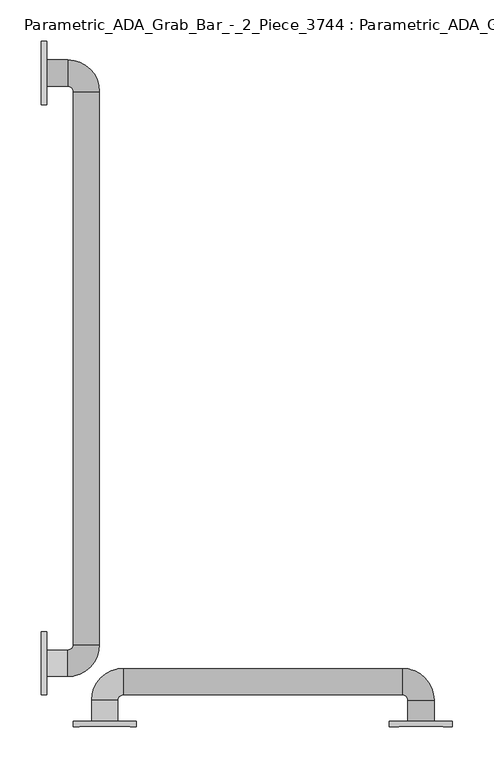
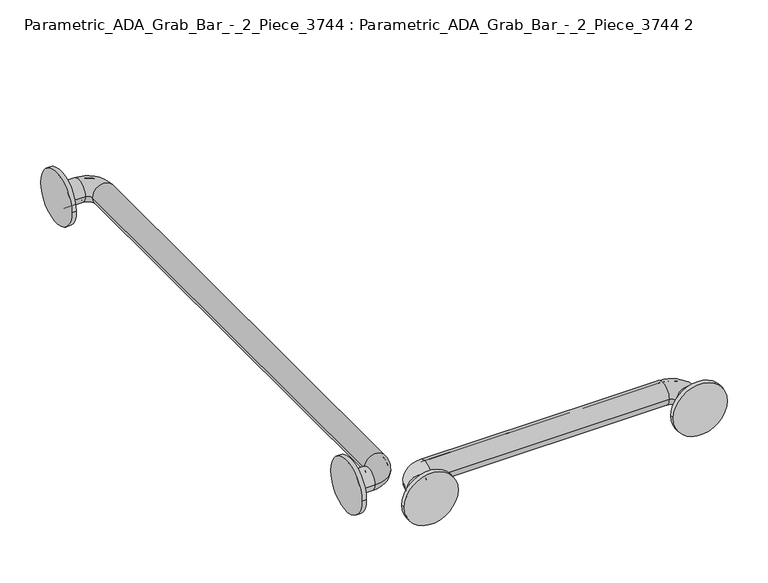
"""IFC4 building model written with IfcOpenShell, lengths in millimetres: proxy geometry, Parametric_ADA_Grab_Bar_-_2_Piece_3744 : Parametric_ADA_Grab_Bar_-_2_Piece_3744 2."""

from ifc_helpers import new_model, si_unit, point, frame, frame_2d, origin, place, context, project, spatial, polyline, circle_curve, ellipse_curve, trimmed, segment, composite_curve, outline, extrude, source, transform, mapped, element, save
from ifc_brep_helpers import plane_surface, cylinder_surface, revolved_surface, advanced_brep


def parametric_ada_grab_bar_2_piece_3744_parametric_ada_grab_bar_cda52879(model_context):
    return source(origin(), model_context, "Body", "SolidModel", [
        advanced_brep(
        [(6.35, 785.01875, 838.2), (6.35, 816.76875, 838.2), (6.35, 788.19375, 838.2), (6.35, 813.59375, 838.2), (31.75, 785.01875, 838.2), (31.75, 816.76875, 838.2), (31.75, 788.19375, 838.2), (31.75, 813.59375, 838.2), (69.85, 778.66875, 838.2), (38.1, 778.66875, 838.2), (66.675, 778.66875, 838.2), (41.275, 778.66875, 838.2), (38.1, 111.91875, 838.2), (69.85, 111.91875, 838.2), (41.275, 111.91875, 838.2), (66.675, 111.91875, 838.2), (31.75, 73.81875, 838.2), (31.75, 105.56875, 838.2), (31.75, 76.99375, 838.2), (31.75, 102.39375, 838.2), (6.35, 105.56875, 838.2), (6.35, 73.81875, 838.2), (6.35, 102.39375, 838.2), (6.35, 76.99375, 838.2)],
        [
            (0, 1, circle_curve(frame((6.35, 800.89375, 838.2), z_axis=(-1.0, 0.0, 0.0), x_axis=(0.0, 1.0, 0.0)), 15.875)),
            (1, 0, circle_curve(frame((6.35, 800.89375, 838.2), z_axis=(-1.0, 0.0, 0.0), x_axis=(0.0, 1.0, 0.0)), 15.875)),
            (2, 3, circle_curve(frame((6.35, 800.89375, 838.2), z_axis=(1.0, 0.0, 0.0), x_axis=(0.0, 1.0, 0.0)), 12.7)),
            (3, 2, circle_curve(frame((6.35, 800.89375, 838.2), z_axis=(1.0, 0.0, 0.0), x_axis=(0.0, 1.0, 0.0)), 12.7)),
            (0, 4),
            (4, 5, circle_curve(frame((31.75, 800.89375, 838.2), z_axis=(-1.0, 0.0, 0.0), x_axis=(0.0, 1.0, 0.0)), 15.875)),
            (5, 1),
            (5, 4, circle_curve(frame((31.75, 800.89375, 838.2), z_axis=(-1.0, 0.0, 0.0), x_axis=(0.0, 1.0, 0.0)), 15.875)),
            (2, 6),
            (6, 7, circle_curve(frame((31.75, 800.89375, 838.2), z_axis=(1.0, 0.0, 0.0), x_axis=(0.0, 1.0, 0.0)), 12.7)),
            (7, 3),
            (7, 6, circle_curve(frame((31.75, 800.89375, 838.2), z_axis=(1.0, 0.0, 0.0), x_axis=(0.0, 1.0, 0.0)), 12.7)),
            (8, 5, circle_curve(frame((31.75, 778.66875, 838.2), z_axis=(0.0, 0.0, 1.0), x_axis=(0.0, 1.0, 0.0)), 38.1)),
            (4, 9, circle_curve(frame((31.75, 778.66875, 838.2), z_axis=(0.0, 0.0, -1.0), x_axis=(0.0, 1.0, 0.0)), 6.35)),
            (9, 8, circle_curve(frame((53.975, 778.66875, 838.2), z_axis=(0.0, 1.0, 0.0), x_axis=(1.0, 0.0, 0.0)), 15.875)),
            (8, 9, circle_curve(frame((53.975, 778.66875, 838.2), z_axis=(0.0, 1.0, 0.0), x_axis=(1.0, 0.0, 0.0)), 15.875)),
            (10, 7, circle_curve(frame((31.75, 778.66875, 838.2), z_axis=(0.0, 0.0, 1.0), x_axis=(0.0, 1.0, 0.0)), 34.925)),
            (6, 11, circle_curve(frame((31.75, 778.66875, 838.2), z_axis=(0.0, 0.0, -1.0), x_axis=(0.0, 1.0, 0.0)), 9.525)),
            (11, 10, circle_curve(frame((53.975, 778.66875, 838.2), z_axis=(0.0, -1.0, 0.0), x_axis=(1.0, 0.0, 0.0)), 12.7)),
            (10, 11, circle_curve(frame((53.975, 778.66875, 838.2), z_axis=(0.0, -1.0, 0.0), x_axis=(1.0, 0.0, 0.0)), 12.7)),
            (9, 12),
            (12, 13, circle_curve(frame((53.975, 111.91875, 838.2), z_axis=(0.0, 1.0, 0.0), x_axis=(1.0, 0.0, 0.0)), 15.875)),
            (13, 8),
            (13, 12, circle_curve(frame((53.975, 111.91875, 838.2), z_axis=(0.0, 1.0, 0.0), x_axis=(1.0, 0.0, 0.0)), 15.875)),
            (11, 14),
            (14, 15, circle_curve(frame((53.975, 111.91875, 838.2), z_axis=(0.0, -1.0, 0.0), x_axis=(1.0, 0.0, 0.0)), 12.7)),
            (15, 10),
            (15, 14, circle_curve(frame((53.975, 111.91875, 838.2), z_axis=(0.0, -1.0, 0.0), x_axis=(1.0, 0.0, 0.0)), 12.7)),
            (16, 13, circle_curve(frame((31.75, 111.91875, 838.2), z_axis=(0.0, 0.0, 1.0), x_axis=(1.0, 0.0, 0.0)), 38.1)),
            (12, 17, circle_curve(frame((31.75, 111.91875, 838.2), z_axis=(0.0, 0.0, -1.0), x_axis=(1.0, 0.0, 0.0)), 6.35)),
            (17, 16, circle_curve(frame((31.75, 89.69375, 838.2), z_axis=(1.0, -1.076610172186615e-12, 0.0), x_axis=(-1.076610172186615e-12, -1.0, 0.0)), 15.875)),
            (16, 17, circle_curve(frame((31.75, 89.69375, 838.2), z_axis=(1.0, 0.0, 0.0), x_axis=(0.0, -1.0, 0.0)), 15.875)),
            (18, 15, circle_curve(frame((31.75, 111.91875, 838.2), z_axis=(0.0, 0.0, 1.0), x_axis=(1.0, 0.0, 0.0)), 34.925)),
            (14, 19, circle_curve(frame((31.75, 111.91875, 838.2), z_axis=(0.0, 0.0, -1.0), x_axis=(1.0, 0.0, 0.0)), 9.525)),
            (19, 18, circle_curve(frame((31.75, 89.69375, 838.2), z_axis=(-1.0, 0.0, 0.0), x_axis=(0.0, -1.0, 0.0)), 12.7)),
            (18, 19, circle_curve(frame((31.75, 89.69375, 838.2), z_axis=(-1.0, 0.0, 0.0), x_axis=(0.0, -1.0, 0.0)), 12.7)),
            (20, 21, circle_curve(frame((6.35, 89.69375, 838.2), z_axis=(-1.0, 0.0, 0.0), x_axis=(0.0, -1.0, 0.0)), 15.875)),
            (21, 20, circle_curve(frame((6.35, 89.69375, 838.2), z_axis=(-1.0, 0.0, 0.0), x_axis=(0.0, -1.0, 0.0)), 15.875)),
            (22, 23, circle_curve(frame((6.35, 89.69375, 838.2), z_axis=(1.0, 0.0, 0.0), x_axis=(0.0, -1.0, 0.0)), 12.7)),
            (23, 22, circle_curve(frame((6.35, 89.69375, 838.2), z_axis=(1.0, 0.0, 0.0), x_axis=(0.0, -1.0, 0.0)), 12.7)),
            (17, 20),
            (21, 16),
            (19, 22),
            (23, 18),
        ],
        [
            plane_surface(frame((6.35, 800.89375, 838.2), z_axis=(-1.0, 0.0, 0.0), x_axis=(0.0, 0.0, 1.0))),
            cylinder_surface(frame((6.35, 800.89375, 838.2), z_axis=(-1.0, 0.0, 0.0), x_axis=(0.0, 1.0, 0.0)), 15.875),
            revolved_surface(polyline([(31.75, 813.59375, 838.2), (6.35, 813.59375, 838.2)]), (6.35, 800.89375, 838.2), (1.0, 0.0, 0.0)),
            revolved_surface(trimmed(ellipse_curve(frame((31.75, 800.89375, 838.2), z_axis=(-1.0, 0.0, 0.0), x_axis=(0.0, 1.0, 0.0)), 15.875, 15.875), [point((31.75, 785.01875, 838.2))], [point((31.75, 816.76875, 838.2))], True, "CARTESIAN"), (31.75, 778.66875, 838.2), (0.0, 0.0, -1.0)),
            revolved_surface(trimmed(ellipse_curve(frame((31.75, 800.89375, 838.2), z_axis=(-1.0, 0.0, 0.0), x_axis=(0.0, 1.0, 0.0)), 15.875, 15.875), [point((31.75, 816.76875, 838.2))], [point((31.75, 785.01875, 838.2))], True, "CARTESIAN"), (31.75, 778.66875, 838.2), (0.0, 0.0, -1.0)),
            revolved_surface(trimmed(ellipse_curve(frame((31.75, 800.89375, 838.2), z_axis=(1.0, 0.0, 0.0), x_axis=(0.0, 1.0, 0.0)), 12.7, 12.7), [point((31.75, 788.19375, 838.2))], [point((31.75, 813.59375, 838.2))], True, "CARTESIAN"), (31.75, 778.66875, 838.2), (0.0, 0.0, -1.0)),
            revolved_surface(trimmed(ellipse_curve(frame((31.75, 800.89375, 838.2), z_axis=(1.0, 0.0, 0.0), x_axis=(0.0, 1.0, 0.0)), 12.7, 12.7), [point((31.75, 813.59375, 838.2))], [point((31.75, 788.19375, 838.2))], True, "CARTESIAN"), (31.75, 778.66875, 838.2), (0.0, 0.0, -1.0)),
            cylinder_surface(frame((53.975, 778.66875, 838.2), z_axis=(0.0, 1.0, 0.0), x_axis=(1.0, 0.0, 0.0)), 15.875),
            revolved_surface(polyline([(66.675, 111.91875000000005, 838.2), (66.675, 778.66875, 838.2)]), (53.975, 778.66875, 838.2), (0.0, -1.0, 0.0)),
            revolved_surface(trimmed(ellipse_curve(frame((53.975, 111.91875, 838.2), z_axis=(0.0, 1.0, 0.0), x_axis=(1.0, 0.0, 0.0)), 15.875, 15.875), [point((38.1, 111.91875, 838.2))], [point((69.85, 111.91875, 838.2))], True, "CARTESIAN"), (31.75, 111.91875, 838.2), (0.0, 0.0, -1.0)),
            revolved_surface(trimmed(ellipse_curve(frame((53.975, 111.91875, 838.2), z_axis=(0.0, 1.0, 0.0), x_axis=(1.0, 0.0, 0.0)), 15.875, 15.875), [point((69.85, 111.91875, 838.2))], [point((38.1, 111.91875, 838.2))], True, "CARTESIAN"), (31.75, 111.91875, 838.2), (0.0, 0.0, -1.0)),
            revolved_surface(trimmed(ellipse_curve(frame((53.975, 111.91875, 838.2), z_axis=(0.0, -1.0, 0.0), x_axis=(1.0, 0.0, 0.0)), 12.7, 12.7), [point((41.275, 111.91875, 838.2))], [point((66.675, 111.91875, 838.2))], True, "CARTESIAN"), (31.75, 111.91875, 838.2), (0.0, 0.0, -1.0)),
            revolved_surface(trimmed(ellipse_curve(frame((53.975, 111.91875, 838.2), z_axis=(0.0, -1.0, 0.0), x_axis=(1.0, 0.0, 0.0)), 12.7, 12.7), [point((66.675, 111.91875, 838.2))], [point((41.275, 111.91875, 838.2))], True, "CARTESIAN"), (31.75, 111.91875, 838.2), (0.0, 0.0, -1.0)),
            plane_surface(frame((6.35, 89.69375, 838.2), z_axis=(-1.0, 0.0, 0.0), x_axis=(0.0, 0.0, 1.0))),
            cylinder_surface(frame((31.75, 89.69375, 838.2), z_axis=(1.0, 0.0, 0.0), x_axis=(0.0, -1.0, 0.0)), 15.875),
            revolved_surface(polyline([(6.350000000000001, 76.99374999999999, 838.2), (31.75, 76.99374999999999, 838.2)]), (31.75, 89.69375, 838.2), (-1.0, 0.0, 0.0)),
        ],
        [
            (0, [[1, 2], [3, 4]]),
            (1, [[-1, 5, 6, 7]]),
            (1, [[-2, -7, 8, -5]]),
            (2, [[-3, 9, 10, 11]]),
            (2, [[-4, -11, 12, -9]]),
            (3, [[13, -6, 14, 15]]),
            (4, [[-14, -8, -13, 16]]),
            (5, [[17, -10, 18, 19]]),
            (6, [[-18, -12, -17, 20]]),
            (7, [[-15, 21, 22, 23]]),
            (7, [[-16, -23, 24, -21]]),
            (8, [[-19, 25, 26, 27]]),
            (8, [[-20, -27, 28, -25]]),
            (9, [[29, -22, 30, 31]]),
            (10, [[-30, -24, -29, 32]]),
            (11, [[33, -26, 34, 35]]),
            (12, [[-34, -28, -33, 36]]),
            (13, [[37, 38], [39, 40]]),
            (14, [[-31, 41, -38, 42]]),
            (14, [[-32, -42, -37, -41]]),
            (15, [[-35, 43, -40, 44]]),
            (15, [[-36, -44, -39, -43]]),
        ],
    ),
        advanced_brep(
        [(92.075, 19.84375, 838.2), (60.325, 19.84375, 838.2), (88.9, 19.84375, 838.2), (63.5, 19.84375, 838.2), (92.075, 45.24375, 838.2), (60.325, 45.24375, 838.2), (88.9, 45.24375, 838.2), (63.5, 45.24375, 838.2), (98.425, 83.34375, 838.2), (98.425, 51.59375, 838.2), (98.425, 80.16875, 838.2), (98.425, 54.76875, 838.2), (434.975, 51.59375, 838.2), (434.975, 83.34375, 838.2), (434.975, 54.76875, 838.2), (434.975, 80.16875, 838.2), (473.075, 45.24375, 838.2), (441.325, 45.24375, 838.2), (469.9, 45.24375, 838.2), (444.5, 45.24375, 838.2), (441.325, 19.84375, 838.2), (473.075, 19.84375, 838.2), (444.5, 19.84375, 838.2), (469.9, 19.84375, 838.2)],
        [
            (0, 1, circle_curve(frame((76.2, 19.84375, 838.2), z_axis=(0.0, -1.0, 0.0), x_axis=(-1.0, 0.0, 0.0)), 15.875)),
            (1, 0, circle_curve(frame((76.2, 19.84375, 838.2), z_axis=(0.0, -1.0, 0.0), x_axis=(-1.0, 0.0, 0.0)), 15.875)),
            (2, 3, circle_curve(frame((76.2, 19.84375, 838.2), z_axis=(0.0, 1.0, 0.0), x_axis=(-1.0, 0.0, 0.0)), 12.7)),
            (3, 2, circle_curve(frame((76.2, 19.84375, 838.2), z_axis=(0.0, 1.0, 0.0), x_axis=(-1.0, 0.0, 0.0)), 12.7)),
            (0, 4),
            (4, 5, circle_curve(frame((76.2, 45.24375, 838.2), z_axis=(0.0, -1.0, 0.0), x_axis=(-1.0, 0.0, 0.0)), 15.875)),
            (5, 1),
            (5, 4, circle_curve(frame((76.2, 45.24375, 838.2), z_axis=(0.0, -1.0, 0.0), x_axis=(-1.0, 0.0, 0.0)), 15.875)),
            (2, 6),
            (6, 7, circle_curve(frame((76.2, 45.24375, 838.2), z_axis=(0.0, 1.0, 0.0), x_axis=(-1.0, 0.0, 0.0)), 12.7)),
            (7, 3),
            (7, 6, circle_curve(frame((76.2, 45.24375, 838.2), z_axis=(0.0, 1.0, 0.0), x_axis=(-1.0, 0.0, 0.0)), 12.7)),
            (8, 5, circle_curve(frame((98.425, 45.24375, 838.2), z_axis=(0.0, 0.0, 1.0), x_axis=(-1.0, 0.0, 0.0)), 38.1)),
            (4, 9, circle_curve(frame((98.425, 45.24375, 838.2), z_axis=(0.0, 0.0, -1.0), x_axis=(-1.0, 0.0, 0.0)), 6.35)),
            (9, 8, circle_curve(frame((98.425, 67.46875, 838.2), z_axis=(-1.0, 0.0, 0.0), x_axis=(0.0, 1.0, 0.0)), 15.875)),
            (8, 9, circle_curve(frame((98.425, 67.46875, 838.2), z_axis=(-1.0, 0.0, 0.0), x_axis=(0.0, 1.0, 0.0)), 15.875)),
            (10, 7, circle_curve(frame((98.425, 45.24375, 838.2), z_axis=(0.0, 0.0, 1.0), x_axis=(-1.0, 0.0, 0.0)), 34.925)),
            (6, 11, circle_curve(frame((98.425, 45.24375, 838.2), z_axis=(0.0, 0.0, -1.0), x_axis=(-1.0, 0.0, 0.0)), 9.525)),
            (11, 10, circle_curve(frame((98.425, 67.46875, 838.2), z_axis=(1.0, 0.0, 0.0), x_axis=(0.0, 1.0, 0.0)), 12.7)),
            (10, 11, circle_curve(frame((98.425, 67.46875, 838.2), z_axis=(1.0, 0.0, 0.0), x_axis=(0.0, 1.0, 0.0)), 12.7)),
            (9, 12),
            (12, 13, circle_curve(frame((434.975, 67.46875, 838.2), z_axis=(-1.0, 0.0, 0.0), x_axis=(0.0, 1.0, 0.0)), 15.875)),
            (13, 8),
            (13, 12, circle_curve(frame((434.975, 67.46875, 838.2), z_axis=(-1.0, 0.0, 0.0), x_axis=(0.0, 1.0, 0.0)), 15.875)),
            (11, 14),
            (14, 15, circle_curve(frame((434.975, 67.46875, 838.2), z_axis=(1.0, 0.0, 0.0), x_axis=(0.0, 1.0, 0.0)), 12.7)),
            (15, 10),
            (15, 14, circle_curve(frame((434.975, 67.46875, 838.2), z_axis=(1.0, 0.0, 0.0), x_axis=(0.0, 1.0, 0.0)), 12.7)),
            (16, 13, circle_curve(frame((434.975, 45.24375, 838.2), z_axis=(0.0, 0.0, 1.0), x_axis=(0.0, 1.0, 0.0)), 38.1)),
            (12, 17, circle_curve(frame((434.975, 45.24375, 838.2), z_axis=(0.0, 0.0, -1.0), x_axis=(0.0, 1.0, 0.0)), 6.35)),
            (17, 16, circle_curve(frame((457.2, 45.24375, 838.2), z_axis=(1.0730574585078145e-12, 1.0, 0.0), x_axis=(1.0, -1.0730574585078145e-12, 0.0)), 15.875)),
            (16, 17, circle_curve(frame((457.2, 45.24375, 838.2), z_axis=(0.0, 1.0, 0.0), x_axis=(1.0, 0.0, 0.0)), 15.875)),
            (18, 15, circle_curve(frame((434.975, 45.24375, 838.2), z_axis=(0.0, 0.0, 1.0), x_axis=(0.0, 1.0, 0.0)), 34.925)),
            (14, 19, circle_curve(frame((434.975, 45.24375, 838.2), z_axis=(0.0, 0.0, -1.0), x_axis=(0.0, 1.0, 0.0)), 9.525)),
            (19, 18, circle_curve(frame((457.2, 45.24375, 838.2), z_axis=(0.0, -1.0, 0.0), x_axis=(1.0, 0.0, 0.0)), 12.7)),
            (18, 19, circle_curve(frame((457.2, 45.24375, 838.2), z_axis=(0.0, -1.0, 0.0), x_axis=(1.0, 0.0, 0.0)), 12.7)),
            (20, 21, circle_curve(frame((457.2, 19.84375, 838.2), z_axis=(0.0, -1.0, 0.0), x_axis=(1.0, 0.0, 0.0)), 15.875)),
            (21, 20, circle_curve(frame((457.2, 19.84375, 838.2), z_axis=(0.0, -1.0, 0.0), x_axis=(1.0, 0.0, 0.0)), 15.875)),
            (22, 23, circle_curve(frame((457.2, 19.84375, 838.2), z_axis=(0.0, 1.0, 0.0), x_axis=(1.0, 0.0, 0.0)), 12.7)),
            (23, 22, circle_curve(frame((457.2, 19.84375, 838.2), z_axis=(0.0, 1.0, 0.0), x_axis=(1.0, 0.0, 0.0)), 12.7)),
            (17, 20),
            (21, 16),
            (19, 22),
            (23, 18),
        ],
        [
            plane_surface(frame((76.2, 19.84375, 838.2), z_axis=(0.0, -1.0, 0.0), x_axis=(0.0, 0.0, 1.0))),
            cylinder_surface(frame((76.2, 19.84375, 838.2), z_axis=(0.0, -1.0, 0.0), x_axis=(-1.0, 0.0, 0.0)), 15.875),
            revolved_surface(polyline([(63.5, 45.24375, 838.2), (63.5, 19.84375, 838.2)]), (76.2, 19.84375, 838.2), (0.0, 1.0, 0.0)),
            revolved_surface(trimmed(ellipse_curve(frame((76.2, 45.24375, 838.2), z_axis=(0.0, -1.0, 0.0), x_axis=(-1.0, 0.0, 0.0)), 15.875, 15.875), [point((92.075, 45.24375, 838.2))], [point((60.325, 45.24375, 838.2))], True, "CARTESIAN"), (98.425, 45.24375, 838.2), (0.0, 0.0, -1.0)),
            revolved_surface(trimmed(ellipse_curve(frame((76.2, 45.24375, 838.2), z_axis=(0.0, -1.0, 0.0), x_axis=(-1.0, 0.0, 0.0)), 15.875, 15.875), [point((60.325, 45.24375, 838.2))], [point((92.075, 45.24375, 838.2))], True, "CARTESIAN"), (98.425, 45.24375, 838.2), (0.0, 0.0, -1.0)),
            revolved_surface(trimmed(ellipse_curve(frame((76.2, 45.24375, 838.2), z_axis=(0.0, 1.0, 0.0), x_axis=(-1.0, 0.0, 0.0)), 12.7, 12.7), [point((88.9, 45.24375, 838.2))], [point((63.5, 45.24375, 838.2))], True, "CARTESIAN"), (98.425, 45.24375, 838.2), (0.0, 0.0, -1.0)),
            revolved_surface(trimmed(ellipse_curve(frame((76.2, 45.24375, 838.2), z_axis=(0.0, 1.0, 0.0), x_axis=(-1.0, 0.0, 0.0)), 12.7, 12.7), [point((63.5, 45.24375, 838.2))], [point((88.9, 45.24375, 838.2))], True, "CARTESIAN"), (98.425, 45.24375, 838.2), (0.0, 0.0, -1.0)),
            cylinder_surface(frame((98.425, 67.46875, 838.2), z_axis=(-1.0, 0.0, 0.0), x_axis=(0.0, 1.0, 0.0)), 15.875),
            revolved_surface(polyline([(434.975, 80.16875, 838.2), (98.425, 80.16875, 838.2)]), (98.425, 67.46875, 838.2), (1.0, 0.0, 0.0)),
            revolved_surface(trimmed(ellipse_curve(frame((434.975, 67.46875, 838.2), z_axis=(-1.0, 0.0, 0.0), x_axis=(0.0, 1.0, 0.0)), 15.875, 15.875), [point((434.975, 51.59375, 838.2))], [point((434.975, 83.34375, 838.2))], True, "CARTESIAN"), (434.975, 45.24375, 838.2), (0.0, 0.0, -1.0)),
            revolved_surface(trimmed(ellipse_curve(frame((434.975, 67.46875, 838.2), z_axis=(-1.0, 0.0, 0.0), x_axis=(0.0, 1.0, 0.0)), 15.875, 15.875), [point((434.975, 83.34375, 838.2))], [point((434.975, 51.59375, 838.2))], True, "CARTESIAN"), (434.975, 45.24375, 838.2), (0.0, 0.0, -1.0)),
            revolved_surface(trimmed(ellipse_curve(frame((434.975, 67.46875, 838.2), z_axis=(1.0, 0.0, 0.0), x_axis=(0.0, 1.0, 0.0)), 12.7, 12.7), [point((434.975, 54.76875, 838.2))], [point((434.975, 80.16875, 838.2))], True, "CARTESIAN"), (434.975, 45.24375, 838.2), (0.0, 0.0, -1.0)),
            revolved_surface(trimmed(ellipse_curve(frame((434.975, 67.46875, 838.2), z_axis=(1.0, 0.0, 0.0), x_axis=(0.0, 1.0, 0.0)), 12.7, 12.7), [point((434.975, 80.16875, 838.2))], [point((434.975, 54.76875, 838.2))], True, "CARTESIAN"), (434.975, 45.24375, 838.2), (0.0, 0.0, -1.0)),
            plane_surface(frame((457.2, 19.84375, 838.2), z_axis=(0.0, -1.0, 0.0), x_axis=(0.0, 0.0, 1.0))),
            cylinder_surface(frame((457.2, 45.24375, 838.2), z_axis=(0.0, 1.0, 0.0), x_axis=(1.0, 0.0, 0.0)), 15.875),
            revolved_surface(polyline([(469.9, 19.84375, 838.2), (469.9, 45.24375, 838.2)]), (457.2, 45.24375, 838.2), (0.0, -1.0, 0.0)),
        ],
        [
            (0, [[1, 2], [3, 4]]),
            (1, [[-1, 5, 6, 7]]),
            (1, [[-2, -7, 8, -5]]),
            (2, [[-3, 9, 10, 11]]),
            (2, [[-4, -11, 12, -9]]),
            (3, [[13, -6, 14, 15]]),
            (4, [[-14, -8, -13, 16]]),
            (5, [[17, -10, 18, 19]]),
            (6, [[-18, -12, -17, 20]]),
            (7, [[-15, 21, 22, 23]]),
            (7, [[-16, -23, 24, -21]]),
            (8, [[-19, 25, 26, 27]]),
            (8, [[-20, -27, 28, -25]]),
            (9, [[29, -22, 30, 31]]),
            (10, [[-30, -24, -29, 32]]),
            (11, [[33, -26, 34, 35]]),
            (12, [[-34, -28, -33, 36]]),
            (13, [[37, 38], [39, 40]]),
            (14, [[-31, 41, -38, 42]]),
            (14, [[-32, -42, -37, -41]]),
            (15, [[-35, 43, -40, 44]]),
            (15, [[-36, -44, -39, -43]]),
        ],
    ),
        extrude(outline(composite_curve([segment(trimmed(circle_curve(frame_2d((89.69375, 838.2)), 38.1), [point((51.59375, 838.2))], [point((127.79375, 838.2))], False, "CARTESIAN"), True, "CONTINUOUS"), segment(trimmed(circle_curve(frame_2d((89.69375, 838.2)), 38.1), [point((127.79375, 838.2))], [point((51.59375, 838.2))], False, "CARTESIAN"), True, "CONTINUOUS")], self_intersect=False)), frame((0.0, 0.0, 0.0), z_axis=(1.0, 0.0, 0.0), x_axis=(0.0, 1.0, 0.0)), (0.0, 0.0, 1.0), 6.35),
        extrude(outline(composite_curve([segment(trimmed(circle_curve(frame_2d((800.89375, 838.2)), 38.1), [point((762.79375, 838.2))], [point((838.99375, 838.2))], False, "CARTESIAN"), True, "CONTINUOUS"), segment(trimmed(circle_curve(frame_2d((800.89375, 838.2)), 38.1), [point((838.99375, 838.2))], [point((762.79375, 838.2))], False, "CARTESIAN"), True, "CONTINUOUS")], self_intersect=False)), frame((0.0, 0.0, 0.0), z_axis=(1.0, 0.0, 0.0), x_axis=(0.0, 1.0, 0.0)), (0.0, 0.0, 1.0), 6.35),
        extrude(outline(composite_curve([segment(trimmed(circle_curve(frame_2d((838.2, 457.2)), 38.1), [point((838.2, 419.1))], [point((838.2, 495.3))], False, "CARTESIAN"), True, "CONTINUOUS"), segment(trimmed(circle_curve(frame_2d((838.2, 457.2)), 38.1), [point((838.2, 495.3))], [point((838.2, 419.1))], False, "CARTESIAN"), True, "CONTINUOUS")], self_intersect=False)), frame((0.0, 13.49375, 0.0), z_axis=(0.0, 1.0, 0.0), x_axis=(0.0, 0.0, 1.0)), (0.0, 0.0, 1.0), 6.35),
        extrude(outline(composite_curve([segment(trimmed(circle_curve(frame_2d((838.2, 76.2)), 38.1), [point((838.2, 38.1))], [point((838.2, 114.3))], False, "CARTESIAN"), True, "CONTINUOUS"), segment(trimmed(circle_curve(frame_2d((838.2, 76.2)), 38.1), [point((838.2, 114.3))], [point((838.2, 38.1))], False, "CARTESIAN"), True, "CONTINUOUS")], self_intersect=False)), frame((0.0, 13.49375, 0.0), z_axis=(0.0, 1.0, 0.0), x_axis=(0.0, 0.0, 1.0)), (0.0, 0.0, 1.0), 6.35),
    ])


if __name__ == "__main__":
    model = new_model("IFC4")
    model_context = context("Model", 3, world=origin())
    ifc_project = project(units=[si_unit("LENGTHUNIT", "METRE", prefix="MILLI")], contexts=[model_context])
    site = spatial("IfcSite", under=ifc_project)
    building = spatial("IfcBuilding", under=site)
    placement = place(None, origin())
    parametric_ada_grab_bar_2_piece_3744_parametric_ada_grab_bar_shape = parametric_ada_grab_bar_2_piece_3744_parametric_ada_grab_bar_cda52879(model_context)
    element("IfcBuildingElementProxy", 1, Name="Parametric_ADA_Grab_Bar_-_2_Piece_3744 : Parametric_ADA_Grab_Bar_-_2_Piece_3744 2", ObjectType="Parametric_ADA_Grab_Bar_-_2_Piece_3744 : Parametric_ADA_Grab_Bar_-_2_Piece_3744 2", at=placement, inside=building, context=model_context, shape_type="MappedRepresentation", body=[
        mapped(parametric_ada_grab_bar_2_piece_3744_parametric_ada_grab_bar_shape, transform((0.0, 0.0, 0.0), x_axis=(1.0, 0.0, 0.0), y_axis=(0.0, 1.0, 0.0), z_axis=(0.0, 0.0, 1.0))),
    ])
    save(model, "model.ifc")

# Revit data of these elements
# Type "Parametric_ADA_Grab_Bar_-_2_Piece_3744 : Parametric_ADA_Grab_Bar_-_2_Piece_3744 2"
#   Keynote = "M10281313.01"
#   Grab bar length (42" min) = 2' - 4"
#   Grab bar height = 2' - 9"
#   Grab bar Length (36" min) = 1' - 3"
#   Face of Wall to Grab bar (6" max) = 0' - 3"
#   Face of Wall to Grab bar (12" max) = 0' - 3"
# Element 1 (IfcBuildingElementProxy, "Parametric_ADA_Grab_Bar_-_2_Piece_3744 : Parametric_ADA_Grab_Bar_-_2_Piece_3744 2")
#   Materials on its faces: "Stainless Steel"
# Materials
#   "Stainless Steel": class "Metal", colour RGB 0 0 0, transparency 0, Description = "Stainless Steel 18/8", Cost = 0
